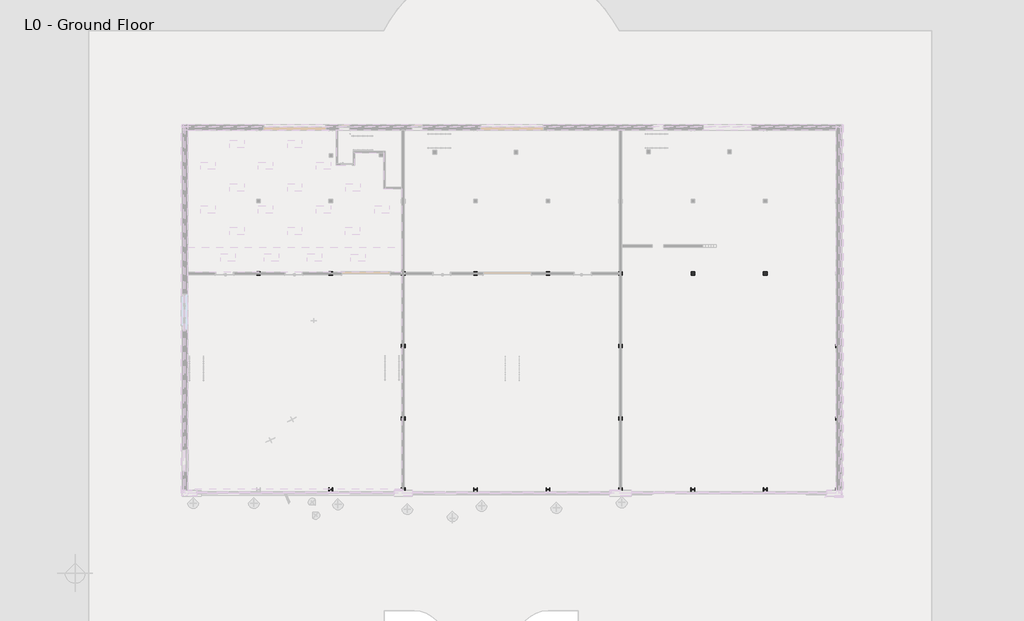
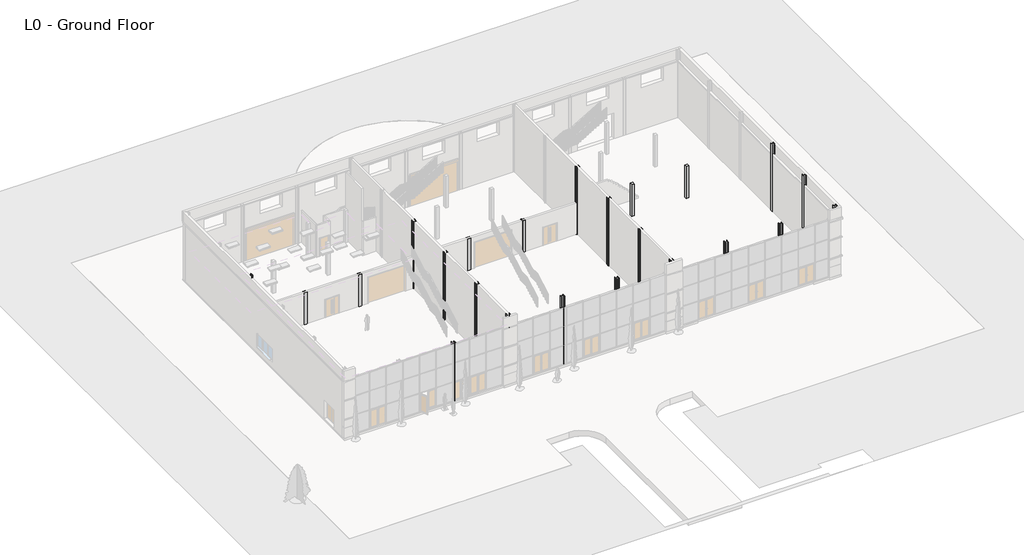
# One storey, part 6 of 14: 23 columns, 22 slabs, 8 footings.
# Revit data of these elements (continued)
# Grids (mm) (continued)
#   "F": line (-7587.705, -22948.762) -> (47341.061, -22948.762)
# Type "Concrete Square : 300 x 300mm"
#   Keynote = "E"
#   b = 300 mm
#   Structural Material [instance default] = Concrete - Cast-in-Place Concrete
# Type "UC-Universal Column-Column : 305x305x97UC"
#   Keynote = "G10"
#   Nominal h = ""
#   W = 0
#   Ix = 0
#   M = 96.9
#   Zx = 0
#   b = 305.3 mm
#   h = 307.9 mm
#   r = 15.2 mm
#   s = 9.9 mm
#   t = 15.4 mm
#   A = 123 m²
#   Structural Material [instance default] = Steel, 45-345
#   Assembly Code = ""
# Type "Pad Foundation-Rectangular : 1000x1000x500"
#   Reinforcement Specs [instance default] = ""
#   Pad Type = "P1"
#   Mesh [instance default] = ""
#   Concrete Grade [instance default] = ""
#   Volume = 0.50 m³
#   Pad Width = 1000 mm
#   Pad Length = 1000 mm
#   Pad Depth = 500 mm
#   Structural Material [instance default] = Concrete - Cast-in-Place Concrete
# Elements 1, 2, 3, 4, 5, 6 (IfcColumn, "Concrete Square : 300 x 300mm")
#   Comments = ""
#   Phase Created = New Construction
#   Materials on its faces: "Concrete - Cast-in-Place Concrete"
# Elements 7, 8, 9, 10, 11, 12, 13, 14, 15, 16, 17, 18, 19, 20, 21, 22, 23 (IfcColumn, "UC-Universal Column-Column : 305x305x97UC")
#   Comments = ""
#   Structural Material = Steel, 45-345
#   Phase Created = New Construction
#   Materials on its faces: "Steel, 45-345"
# Elements 24, 25, 26, 27, 28, 29 (IfcFooting, "Wall Foundation - Commercial 1300 x 450")
#   Phase Created = New Construction
#   Materials on its faces: "Concrete, Cast In Situ"
# Elements 30, 31 (IfcFooting, "Wall Foundation - Commercial 1300 x 450")
#   Comments = ""
#   Phase Created = New Construction
#   Materials on its faces: "Concrete, Cast In Situ"
# Elements 32, 33, 34, 35, 36, 37, 38, 39, 40, 41, 42, 43, 44, 45, 46, 47, 48, 49, 50, 51, 52, 53 (IfcSlab, "Pad Foundation-Rectangular : 1000x1000x500")
#   Comments = ""
#   Reinforcement Specs = ""
#   Mesh = ""
#   Concrete Grade = ""
#   Structural Material = Concrete - Cast-in-Place Concrete
#   Phase Created = New Construction
#   Materials on its faces: "Concrete - Cast-in-Place Concrete"
# Materials
#   "Concrete - Cast-in-Place Concrete": class "Concrete", colour RGB 192 192 192, transparency 0
#   "Steel, 45-345": class "Metal", colour RGB 247 247 247, transparency 0, Description = "Steel 345 MPa", Cost = 0
#   "Concrete, Cast In Situ": class "Concrete", colour RGB 192 192 192, transparency 0, Description = "physical material", Cost = 0
# Room at (37819.631, -8755.145) mm, phase "New Construction", upper level "L0 - Ground Floor", upper offset 4000 mm, lower offset 0 mm
#   Number = "5"
#   Name = "Unit 3"
# Room at (19838.479, -14949.994) mm, phase "New Construction", upper level "L0 - Ground Floor", upper offset 4000 mm, lower offset 0 mm
#   Number = "3"
#   Name = "Showroom"
# Room at (19838.479, 1158.704) mm, phase "New Construction", upper level "L0 - Ground Floor", upper offset 4000 mm, lower offset 0 mm
#   Number = "4"
#   Name = "STORAGE / DISPATCH AREA"
# Room at (2534.039, 34.316) mm, phase "New Construction", upper level "L0 - Ground Floor", upper offset 4000 mm, lower offset 0 mm
#   Number = "1"
#   Name = "STORAGE / DISPATCH AREA"
#   Include In Daylighting = yes
#   Automated Shades = no
# Room at (2390.683, -14731.423) mm, phase "New Construction", upper level "L0 - Ground Floor", upper offset 4000 mm, lower offset 0 mm
#   Number = "2"
#   Name = "Showroom"
#   Include In Daylighting = yes
#   Automated Shades = no
